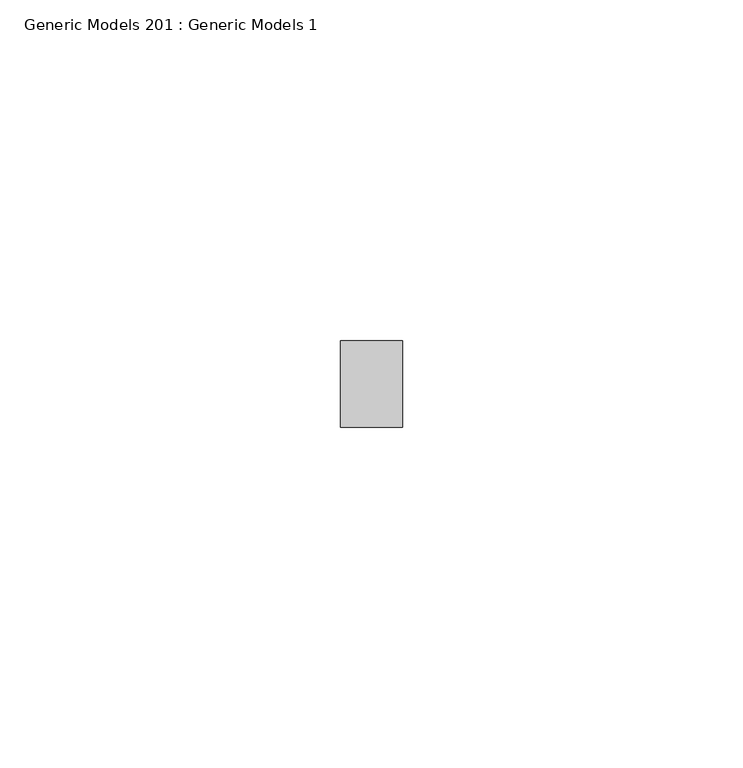
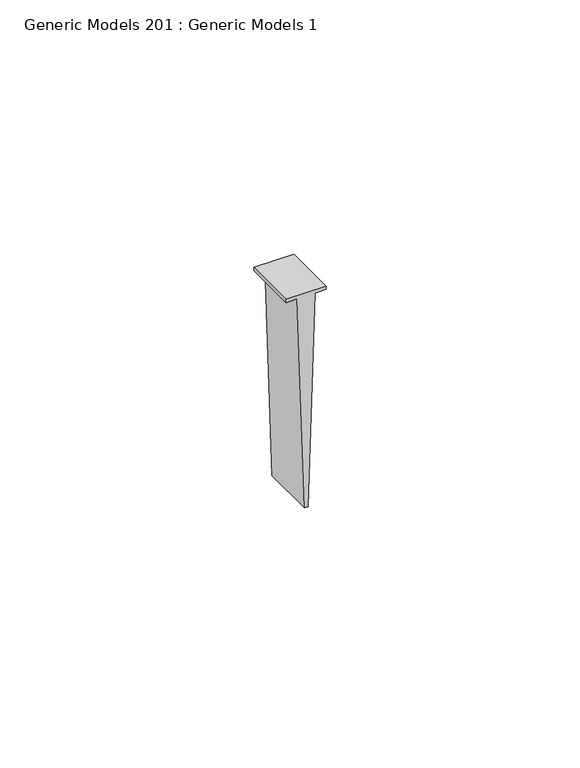
"""IFC4 building model written with IfcOpenShell, lengths in millimetres: proxy geometry, Generic Models 201 : Generic Models 1."""

from ifc_helpers import new_model, si_unit, frame, origin, place, context, project, spatial, polyline, outline, extrude, source, transform, mapped, element, save


def generic_models_201_generic_models_1_6cd63f98(model_context):
    return source(origin(), model_context, "Body", "SweptSolid", [
        extrude(outline(polyline([(2.38125, 49733.4159), (1.5875, 49733.4159), (1.5875, 49735.9657636), (-49.2125, 49737.5631527), (-49.2125, 49738.3618473), (1.5875, 49739.9592364), (1.5875, 49742.5091), (2.38125, 49742.5091), (2.38125, 49733.4159)])), frame((0.0, 565.15, 0.0), z_axis=(0.0, 1.0, 0.0), x_axis=(0.0, 0.0, 1.0)), (0.0, 0.0, 1.0), 12.7),
    ])


if __name__ == "__main__":
    model = new_model("IFC4")
    model_context = context("Model", 3, world=origin())
    ifc_project = project(units=[si_unit("LENGTHUNIT", "METRE", prefix="MILLI")], contexts=[model_context])
    site = spatial("IfcSite", under=ifc_project)
    building = spatial("IfcBuilding", under=site)
    placement = place(None, origin())
    generic_models_201_generic_models_1_shape = generic_models_201_generic_models_1_6cd63f98(model_context)
    element("IfcBuildingElementProxy", 1, Name="Generic Models 201 : Generic Models 1", ObjectType="Generic Models 201 : Generic Models 1", at=placement, inside=building, context=model_context, shape_type="MappedRepresentation", body=[
        mapped(generic_models_201_generic_models_1_shape, transform((0.0, 0.0, 0.0), x_axis=(1.0, 0.0, 0.0), y_axis=(0.0, 1.0, 0.0), z_axis=(0.0, 0.0, 1.0))),
    ])
    save(model, "model.ifc")

# Revit data of these elements
# Element 1 (IfcBuildingElementProxy, "Generic Models 201 : Generic Models 1")
#   Materials on its faces: "METAL RUNNER CHANNEL; FASTEN @ 24\" O.C."
# Materials
#   "METAL RUNNER CHANNEL; FASTEN @ 24\" O.C.": class "Unassigned", colour RGB 210 209 208, transparency 0, Keynote = "M05121300.02", Cost = 0
